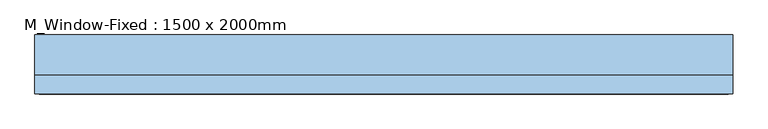
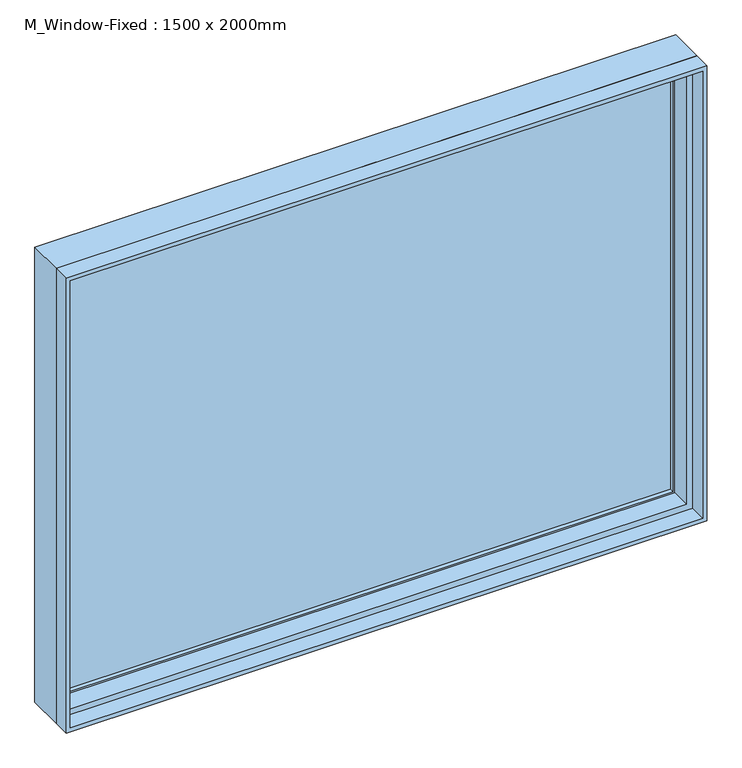
"""IFC4 building model written with IfcOpenShell, lengths in millimetres: window geometry, M_Window-Fixed : 1500 x 2000mm."""

from ifc_helpers import new_model, si_unit, frame, origin, place, context, project, spatial, polyline, outline, extrude, faceted_brep, source, transform, mapped, element, save


def m_window_fixed_1500_x_2000mm_d3dd2c19(model_context):
    return source(origin(), model_context, "Body", "SolidModel", [
        faceted_brep([(1000.0, -20.25, 2400.0), (1000.0, 94.05, 2400.0), (-1000.0, 94.05, 2400.0), (-1000.0, -20.25, 2400.0), (-1000.0, 94.05, 900.0), (-1000.0, -20.25, 900.0), (1000.0, 94.05, 900.0), (1000.0, -20.25, 900.0), (968.25, -20.25, 2368.25), (968.25, -20.25, 931.75), (-968.25, -20.25, 931.75), (-968.25, -20.25, 2368.25), (-987.3, 94.05, 2387.3), (-987.3, 94.05, 912.7), (987.3, 94.05, 912.7), (987.3, 94.05, 2387.3), (968.25, 43.25, 2368.25), (-968.25, 43.25, 2368.25), (987.3, 43.25, 2387.3), (-987.3, 43.25, 2387.3), (-968.25, 43.25, 931.75), (-987.3, 43.25, 912.7), (968.25, 43.25, 931.75), (987.3, 43.25, 912.7)], [[[0, 1, 2, 3]], [[3, 2, 4, 5]], [[5, 4, 6, 7]], [[3, 5, 7, 0], [8, 9, 10, 11]], [[7, 6, 1, 0]], [[1, 6, 4, 2], [12, 13, 14, 15]], [[16, 8, 11, 17]], [[15, 18, 19, 12]], [[17, 11, 10, 20]], [[12, 19, 21, 13]], [[20, 10, 9, 22]], [[13, 21, 23, 14]], [[22, 9, 8, 16]], [[18, 23, 21, 19], [17, 20, 22, 16]], [[14, 23, 18, 15]]]),
        extrude(outline(polyline([(2400.0, -1000.0), (900.0, -1000.0), (900.0, 1000.0), (2400.0, 1000.0), (2400.0, -1000.0)]), holes=[polyline([(2387.3, 987.3), (912.7, 987.3), (912.7, -987.3), (2387.3, -987.3), (2387.3, 987.3)])]), frame((0.0, -75.0, 0.0), z_axis=(0.0, 1.0, 0.0), x_axis=(0.0, 0.0, 1.0)), (0.0, 0.0, 1.0), 54.75),
        extrude(outline(polyline([(912.7, 987.3), (2387.3, 987.3), (2387.3, -987.3), (912.7, -987.3), (912.7, 987.3)]), holes=[polyline([(938.1, -961.9), (2361.9, -961.9), (2361.9, 961.9), (938.1, 961.9), (938.1, -961.9)])]), frame((0.0, 43.25, 0.0), z_axis=(0.0, 1.0, 0.0), x_axis=(0.0, 0.0, 1.0)), (0.0, 0.0, 1.0), 44.45),
        extrude(outline(polyline([(961.9, 75.0), (961.9, 68.65), (-961.9, 68.65), (-961.9, 75.0), (961.9, 75.0)])), frame((0.0, 0.0, 938.1), z_axis=(0.0, 0.0, 1.0), x_axis=(1.0, 0.0, 0.0)), (0.0, 0.0, 1.0), 1423.8),
        extrude(outline(polyline([(-961.9, 55.95), (-961.9, 62.3), (961.9, 62.3), (961.9, 55.95), (-961.9, 55.95)])), frame((0.0, 0.0, 938.1), z_axis=(0.0, 0.0, 1.0), x_axis=(1.0, 0.0, 0.0)), (0.0, 0.0, 1.0), 1423.8),
    ])


if __name__ == "__main__":
    model = new_model("IFC4")
    model_context = context("Model", 3, world=origin())
    ifc_project = project(units=[si_unit("LENGTHUNIT", "METRE", prefix="MILLI")], contexts=[model_context])
    site = spatial("IfcSite", under=ifc_project)
    building = spatial("IfcBuilding", under=site)
    placement = place(None, origin())
    m_window_fixed_1500_x_2000mm_shape = m_window_fixed_1500_x_2000mm_d3dd2c19(model_context)
    element("IfcWindow", 1, ObjectType="M_Window-Fixed : 1500 x 2000mm", at=placement, inside=building, context=model_context, shape_type="MappedRepresentation", body=[
        mapped(m_window_fixed_1500_x_2000mm_shape, transform((0.0, 0.0, 0.0), x_axis=(1.0, 0.0, 0.0), y_axis=(0.0, 1.0, 0.0), z_axis=(0.0, 0.0, 1.0))),
    ])
    save(model, "model.ifc")

# Revit data of these elements
# Type "M_Window-Fixed : 1500 x 2000mm"
#   Type Mark = "43"
#   Fire Rating = "0.5h"
#   Assembly Code = "B2020100"
#   Analytic Construction = "Double glazing - domestic"
#   Window Inset [instance default] = 0 mm
#   Wall Thickness [instance default] = 150 mm
#   Visual Light Transmittance = 0.81
#   Thermal Resistance (R) = 0.319569 (m²·K)/W
#   Solar Heat Gain Coefficient = 0.76
#   Rough Width = 2015 mm
#   Rough Height = 1515 mm
#   Interior Wall Closure [instance default] = 54.75 mm
#   Height = 1500 mm
#   Heat Transfer Coefficient (U) = 3.12929 W/(m²·K)
#   Frame Extension [instance default] = 6.35 mm
#   Exterior Wall Closure [instance default] = 31.75 mm
#   Extension Jamb [instance default] = 54.75 mm
#   Default Sill Height = 900 mm
#   Width = 2000 mm
#   Muntin Visibility = yes
#   Interior Trim Visibility [instance default] = yes
#   Exterior Trim Visibility [instance default] = yes
#   Extension Jamb Visibility [instance default] = yes
#   Muntin Pattern = M_Muntin Pattern_2x2 : M_Muntin Pattern_2x2
#   Interior Trim Material = Wood - Stained
#   Interior Trim = M_Trim-Window-Interior-Flat : Picture Frame
#   Interior Frame Material = Wood - Stained
#   Glass Panel Material = Glass
#   Exterior Trim Material = Clad - White
#   Exterior Trim = M_Trim-Window-Exterior-Flat : with Sill
#   Exterior Frame Material = Clad - White
#   Wall Closure = (empty or 0)
# Element 1 (IfcWindow, "M_Window-Fixed : 1500 x 2000mm")
#   Materials on its faces: "Wood - Stained", "Glass", "Clad - White"
# Materials
#   "Wood - Stained": class "Wood", colour RGB 173 132 96, transparency 0, Cost = 0
#   "Glass": class "Glass", colour RGB 245 245 243, transparency 1, Description = "Soda Lime Glass", Cost = 0
#   "Clad - White": class "Wood", colour RGB 245 245 243, transparency 0, Cost = 0
